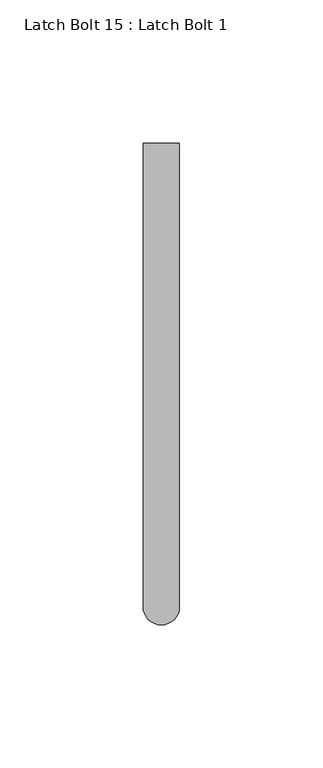
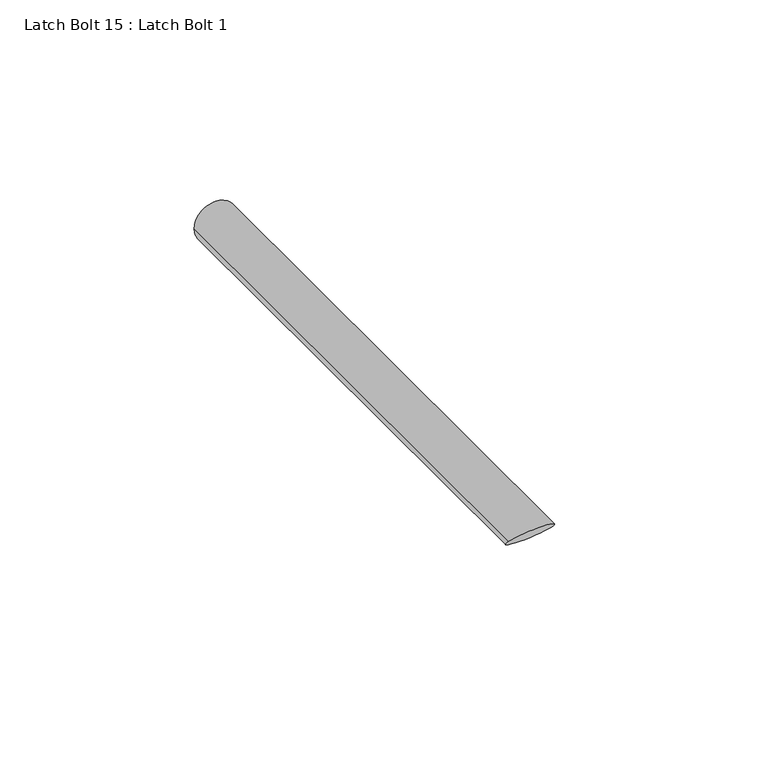
"""IFC4 building model written with IfcOpenShell, lengths in millimetres: proxy geometry, Latch Bolt 15 : Latch Bolt 1."""

from ifc_helpers import new_model, si_unit, frame, origin, place, context, project, spatial, circle_curve, ellipse_curve, source, transform, mapped, element, save
from ifc_brep_helpers import plane_surface, cylinder_surface, advanced_brep


def latch_bolt_15_latch_bolt_1_cfdedea9(model_context):
    return source(origin(), model_context, "Body", "AdvancedBrep", [
        advanced_brep(
        [(587306.3685739, -535131.7163841, 1066.8), (587319.0685739, -535131.7163841, 1066.8), (587306.3685739, -535293.6413841, 1066.8), (587312.7185739, -535299.9913841, 1073.15), (587319.0685739, -535293.6413841, 1066.8)],
        [
            (0, 1, circle_curve(frame((587312.7185739, -535131.7163841, 1066.8), z_axis=(0.0, 1.0, 0.0), x_axis=(1.0, 0.0, 0.0)), 6.35)),
            (1, 0, circle_curve(frame((587312.7185739, -535131.7163841, 1066.8), z_axis=(0.0, 1.0, 0.0), x_axis=(1.0, 0.0, 0.0)), 6.35)),
            (0, 2),
            (2, 3, ellipse_curve(frame((587312.7185739, -535293.6413841, 1066.8), z_axis=(0.0, 0.7071067811870104, 0.7071067811860847), x_axis=(0.0, 0.7071067811860846, -0.7071067811870104)), 8.9802561, 6.35)),
            (3, 4, ellipse_curve(frame((587312.7185739, -535293.6413841, 1066.8), z_axis=(0.0, 0.7071067811870104, 0.7071067811860847), x_axis=(0.0, 0.7071067811860846, -0.7071067811870104)), 8.9802561, 6.35)),
            (4, 1),
            (4, 2, ellipse_curve(frame((587312.7185739, -535293.6413841, 1066.8), z_axis=(0.0, 0.7071067811870104, 0.7071067811860847), x_axis=(0.0, 0.7071067811860846, -0.7071067811870104)), 8.9802561, 6.35)),
        ],
        [
            plane_surface(frame((587319.0685739, -535131.7163841, 1066.8), z_axis=(0.0, 1.0, 0.0), x_axis=(0.0, 0.0, -1.0))),
            cylinder_surface(frame((587312.7185739, -535299.9913841, 1066.8), z_axis=(0.0, 1.0, 0.0), x_axis=(1.0, 0.0, 0.0)), 6.35),
            plane_surface(frame((587338.1185739, -535284.1163841, 1057.275), z_axis=(0.0, -0.7071067811870104, -0.7071067811860847), x_axis=(-1.0, 0.0, 0.0))),
        ],
        [
            (0, [[1, 2]]),
            (1, [[-1, 3, 4, 5, 6]]),
            (1, [[-2, -6, 7, -3]]),
            (2, [[-4, -7, -5]]),
        ],
    ),
    ])


if __name__ == "__main__":
    model = new_model("IFC4")
    model_context = context("Model", 3, world=origin())
    ifc_project = project(units=[si_unit("LENGTHUNIT", "METRE", prefix="MILLI")], contexts=[model_context])
    site = spatial("IfcSite", under=ifc_project)
    building = spatial("IfcBuilding", under=site)
    placement = place(None, origin())
    latch_bolt_15_latch_bolt_1_shape = latch_bolt_15_latch_bolt_1_cfdedea9(model_context)
    element("IfcBuildingElementProxy", 1, Name="Latch Bolt 15 : Latch Bolt 1", ObjectType="Latch Bolt 15 : Latch Bolt 1", at=placement, inside=building, context=model_context, shape_type="MappedRepresentation", body=[
        mapped(latch_bolt_15_latch_bolt_1_shape, transform((0.0, 0.0, 0.0), x_axis=(1.0, 0.0, 0.0), y_axis=(0.0, 1.0, 0.0), z_axis=(0.0, 0.0, 1.0))),
    ])
    save(model, "model.ifc")

# Revit data of these elements
# Element 1 (IfcBuildingElementProxy, "Latch Bolt 15 : Latch Bolt 1")
#   Materials on its faces: "GALV. GATE LATCH"
# Materials
#   "GALV. GATE LATCH": class "Metal", colour RGB 189 187 185, transparency 0, Description = "Carbon steel", Cost = 0
